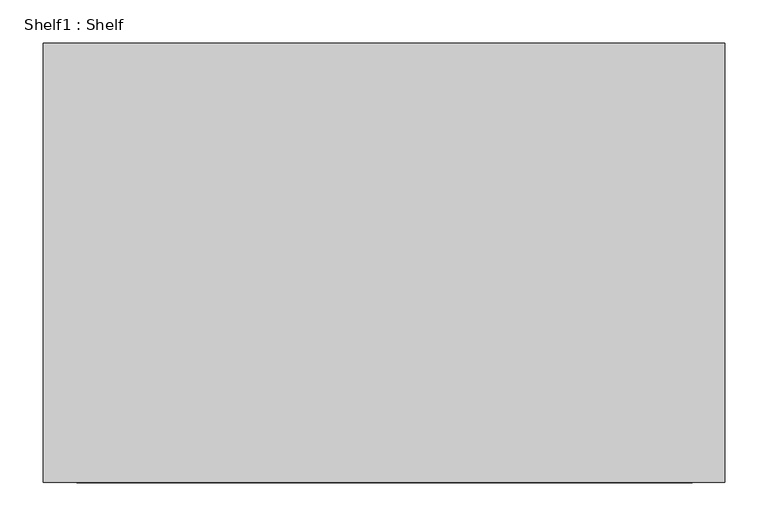
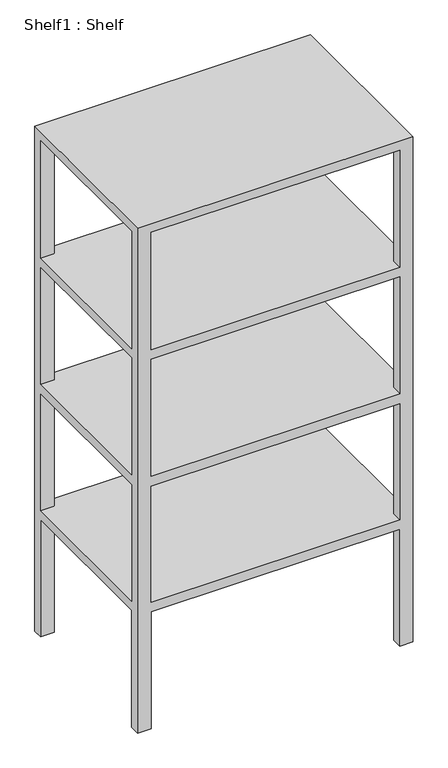
"""IFC4 building model written with IfcOpenShell, lengths in millimetres: furniture geometry, Shelf1 : Shelf."""

from ifc_helpers import new_model, si_unit, origin, place, context, project, spatial, faceted_brep, source, transform, mapped, element, save


def shelf1_shelf_c8367ec8(model_context):
    return source(origin(), model_context, "Body", "Brep", [
        faceted_brep([(14906.8798744, 3328.6615366, 1524.0), (14119.4798744, 3328.6615366, 1524.0), (14119.4798744, 2820.6615366, 1524.0), (14906.8798744, 2820.6615366, 1524.0), (14906.8798744, 2849.585331, 0.0), (14906.8798744, 2820.6615366, 0.0), (14869.5001442, 2820.6615366, 0.0), (14869.5001442, 2849.585331, 0.0), (14906.8798744, 3328.6615366, 0.0), (14906.8798744, 3299.6392676, 0.0), (14869.5001442, 3299.6392676, 0.0), (14869.5001442, 3328.6615366, 0.0), (14158.3001442, 2820.6615366, 0.0), (14119.4798744, 2820.6615366, 0.0), (14119.4798744, 2849.585331, 0.0), (14158.3001442, 2849.585331, 0.0), (14119.4798744, 3299.6392676, 0.0), (14119.4798744, 3328.6615366, 0.0), (14158.3001442, 3328.6615366, 0.0), (14158.3001442, 3299.6392676, 0.0), (14869.5001442, 3328.6615366, 353.3332002), (14158.3001442, 3328.6615366, 353.3332002), (14869.5001442, 3328.6615366, 1497.6781444), (14158.3001442, 3328.6615366, 1497.6781444), (14158.3001442, 3328.6615366, 1143.0), (14869.5001442, 3328.6615366, 1143.0), (14869.5001442, 3328.6615366, 1114.8196695), (14158.3001442, 3328.6615366, 1114.8196695), (14158.3001442, 3328.6615366, 762.0), (14869.5001442, 3328.6615366, 762.0), (14869.5001442, 3328.6615366, 731.9611947), (14158.3001442, 3328.6615366, 731.9611947), (14158.3001442, 3328.6615366, 381.0), (14869.5001442, 3328.6615366, 381.0), (14119.4798744, 3299.6392676, 353.3332002), (14119.4798744, 2849.585331, 353.3332002), (14119.4798744, 3300.0671384, 1497.6781444), (14119.4798744, 2849.585331, 1497.6781444), (14119.4798744, 2849.585331, 1143.0), (14119.4798744, 3300.0671384, 1143.0), (14119.4798744, 3299.6392676, 1114.8196695), (14119.4798744, 2849.585331, 1114.8196695), (14119.4798744, 2849.585331, 762.0), (14119.4798744, 3299.6392676, 762.0), (14119.4798744, 3299.6392676, 731.9611947), (14119.4798744, 2849.585331, 731.9611947), (14119.4798744, 2849.585331, 381.0), (14119.4798744, 3299.6392676, 381.0), (14158.3001442, 2820.6615366, 353.3332002), (14869.5001442, 2820.6615366, 353.3332002), (14158.3001442, 2820.6615366, 1497.6781444), (14869.5001442, 2820.6615366, 1497.6781444), (14869.5001442, 2820.6615366, 1143.0), (14158.3001442, 2820.6615366, 1143.0), (14158.3001442, 2820.6615366, 1114.8196695), (14869.5001442, 2820.6615366, 1114.8196695), (14869.5001442, 2820.6615366, 762.0), (14158.3001442, 2820.6615366, 762.0), (14158.3001442, 2820.6615366, 731.9611947), (14869.5001442, 2820.6615366, 731.9611947), (14869.5001442, 2820.6615366, 381.0), (14158.3001442, 2820.6615366, 381.0), (14906.8798744, 2849.585331, 353.3332002), (14906.8798744, 3299.6392676, 353.3332002), (14906.8798744, 2849.585331, 1497.6781444), (14906.8798744, 3299.6392676, 1497.6781444), (14906.8798744, 3299.6392676, 1143.0), (14906.8798744, 2849.585331, 1143.0), (14906.8798744, 2849.585331, 1114.8196695), (14906.8798744, 3299.6392676, 1114.8196695), (14906.8798744, 3299.6392676, 762.0), (14906.8798744, 2849.585331, 762.0), (14906.8798744, 2849.585331, 731.9611947), (14906.8798744, 3299.6392676, 731.9611947), (14906.8798744, 3299.6392676, 381.0), (14906.8798744, 2849.585331, 381.0), (14158.3001442, 2849.585331, 1497.6781444), (14158.3001442, 3300.0671384, 1497.6781444), (14869.5001442, 3299.6392676, 1497.6781444), (14869.5001442, 2849.585331, 1497.6781444), (14158.3001442, 2849.585331, 1143.0), (14869.5001442, 2849.585331, 1143.0), (14869.5001442, 3299.6392676, 1143.0), (14158.3001442, 3300.0671384, 1143.0), (14158.3001442, 2849.585331, 1114.8196695), (14158.3001442, 3299.6392676, 1114.8196695), (14869.5001442, 3299.6392676, 1114.8196695), (14869.5001442, 2849.585331, 1114.8196695), (14158.3001442, 2849.585331, 762.0), (14869.5001442, 2849.585331, 762.0), (14869.5001442, 3299.6392676, 762.0), (14158.3001442, 3299.6392676, 762.0), (14158.3001442, 2849.585331, 731.9611947), (14158.3001442, 3299.6392676, 731.9611947), (14869.5001442, 3299.6392676, 731.9611947), (14869.5001442, 2849.585331, 731.9611947), (14158.3001442, 2849.585331, 381.0), (14869.5001442, 2849.585331, 381.0), (14869.5001442, 3299.6392676, 381.0), (14158.3001442, 3299.6392676, 381.0), (14158.3001442, 2849.585331, 353.3332002), (14158.3001442, 3299.6392676, 353.3332002), (14869.5001442, 3299.6392676, 353.3332002), (14869.5001442, 2849.585331, 353.3332002)], [[[0, 1, 2, 3]], [[4, 5, 6, 7]], [[8, 9, 10, 11]], [[12, 13, 14, 15]], [[16, 17, 18, 19]], [[1, 0, 8, 11, 20, 21, 18, 17], [22, 23, 24, 25], [26, 27, 28, 29], [30, 31, 32, 33]], [[2, 1, 17, 16, 34, 35, 14, 13], [36, 37, 38, 39], [40, 41, 42, 43], [44, 45, 46, 47]], [[3, 2, 13, 12, 48, 49, 6, 5], [50, 51, 52, 53], [54, 55, 56, 57], [58, 59, 60, 61]], [[0, 3, 5, 4, 62, 63, 9, 8], [64, 65, 66, 67], [68, 69, 70, 71], [72, 73, 74, 75]], [[76, 37, 36, 77, 23, 22, 78, 65, 64, 79, 51, 50]], [[80, 53, 52, 81, 67, 66, 82, 25, 24, 83, 39, 38]], [[76, 50, 53, 80]], [[51, 79, 81, 52]], [[79, 64, 67, 81]], [[65, 78, 82, 66]], [[78, 22, 25, 82]], [[23, 77, 83, 24]], [[77, 36, 39, 83]], [[37, 76, 80, 38]], [[84, 41, 40, 85, 27, 26, 86, 69, 68, 87, 55, 54]], [[88, 57, 56, 89, 71, 70, 90, 29, 28, 91, 43, 42]], [[84, 54, 57, 88]], [[55, 87, 89, 56]], [[87, 68, 71, 89]], [[69, 86, 90, 70]], [[86, 26, 29, 90]], [[27, 85, 91, 28]], [[85, 40, 43, 91]], [[41, 84, 88, 42]], [[92, 45, 44, 93, 31, 30, 94, 73, 72, 95, 59, 58]], [[96, 61, 60, 97, 75, 74, 98, 33, 32, 99, 47, 46]], [[92, 58, 61, 96]], [[59, 95, 97, 60]], [[95, 72, 75, 97]], [[73, 94, 98, 74]], [[94, 30, 33, 98]], [[31, 93, 99, 32]], [[93, 44, 47, 99]], [[45, 92, 96, 46]], [[100, 35, 34, 101, 21, 20, 102, 63, 62, 103, 49, 48]], [[100, 48, 12, 15]], [[49, 103, 7, 6]], [[103, 62, 4, 7]], [[63, 102, 10, 9]], [[102, 20, 11, 10]], [[21, 101, 19, 18]], [[101, 34, 16, 19]], [[35, 100, 15, 14]]]),
    ])


if __name__ == "__main__":
    model = new_model("IFC4")
    model_context = context("Model", 3, world=origin())
    ifc_project = project(units=[si_unit("LENGTHUNIT", "METRE", prefix="MILLI")], contexts=[model_context])
    site = spatial("IfcSite", under=ifc_project)
    building = spatial("IfcBuilding", under=site)
    placement = place(None, origin())
    shelf1_shelf_shape = shelf1_shelf_c8367ec8(model_context)
    element("IfcFurniture", 1, ObjectType="Shelf1 : Shelf", at=placement, inside=building, context=model_context, shape_type="MappedRepresentation", body=[
        mapped(shelf1_shelf_shape, transform((0.0, 0.0, 0.0), x_axis=(1.0, 0.0, 0.0), y_axis=(0.0, 1.0, 0.0), z_axis=(0.0, 0.0, 1.0))),
    ])
    save(model, "model.ifc")

# Revit data of these elements
# Element 1 (IfcFurniture, "Shelf1 : Shelf")
#   Materials on its faces: "food"
# Materials
#   "food": class "Glass", colour RGB 233 233 233, transparency 0, Description = "Soda Lime Glass", Cost = 0
